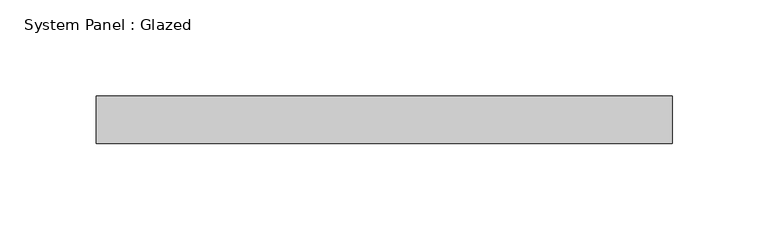
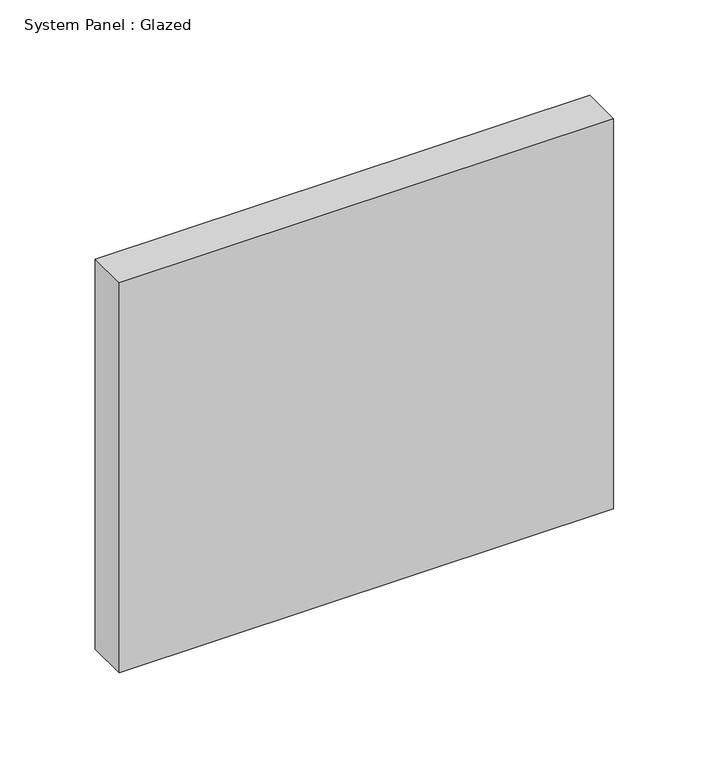
"""IFC4 building model written with IfcOpenShell, lengths in millimetres: plate geometry, System Panel : Glazed."""

from ifc_helpers import new_model, si_unit, origin, origin_with_axes, place, context, project, spatial, polyline, outline, extrude, source, transform, mapped, element, save


def system_panel_glazed_02a4bfdf(model_context):
    return source(origin(), model_context, "Body", "SweptSolid", [
        extrude(outline(polyline([(150.0, 24.5), (-150.0, 24.5), (-150.0, 49.5), (150.0, 49.5), (150.0, 24.5)])), origin_with_axes(), (0.0, 0.0, 1.0), 250.0),
    ])


if __name__ == "__main__":
    model = new_model("IFC4")
    model_context = context("Model", 3, world=origin())
    ifc_project = project(units=[si_unit("LENGTHUNIT", "METRE", prefix="MILLI")], contexts=[model_context])
    site = spatial("IfcSite", under=ifc_project)
    building = spatial("IfcBuilding", under=site)
    placement = place(None, origin())
    system_panel_glazed_shape = system_panel_glazed_02a4bfdf(model_context)
    element("IfcPlate", 1, ObjectType="System Panel : Glazed", at=placement, inside=building, context=model_context, shape_type="MappedRepresentation", body=[
        mapped(system_panel_glazed_shape, transform((0.0, 0.0, 0.0), x_axis=(1.0, 0.0, 0.0), y_axis=(0.0, 1.0, 0.0), z_axis=(0.0, 0.0, 1.0))),
    ])
    save(model, "model.ifc")

# Revit data of these elements
# Element 1 (IfcPlate, "System Panel : Glazed")
#   Materials on its faces: "Glass"
# Materials
#   "Glass": class "Glass", colour RGB 218 227 224, transparency 0.85, Description = "Soda Lime Glass", Cost = 0
